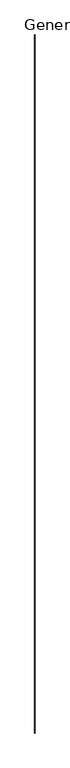
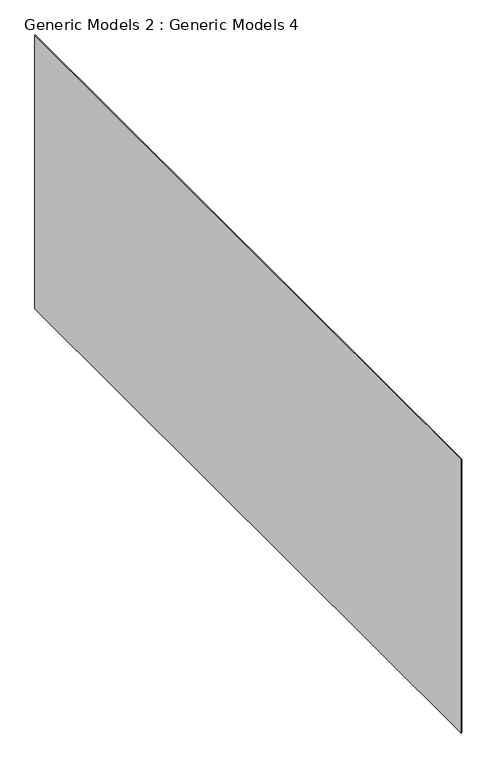
"""IFC4 building model written with IfcOpenShell, lengths in millimetres: proxy geometry, Generic Models 2 : Generic Models 4."""

from ifc_helpers import new_model, si_unit, frame, origin, place, context, project, spatial, polyline, outline, extrude, source, transform, mapped, element, save


def generic_models_2_generic_models_4_d4be96ae(model_context):
    return source(origin(), model_context, "Body", "SweptSolid", [
        extrude(outline(polyline([(593591.3576893, -527524.3545647), (593591.3576893, -584979.050959), (593565.9576893, -584979.050959), (593565.9576893, -527524.3545647), (593591.3576893, -527524.3545647)])), frame((0.0, 0.0, -2503.337634), z_axis=(0.0, 0.0, 1.0), x_axis=(1.0, 0.0, 0.0)), (0.0, 0.0, 1.0), 22488.6259865),
    ])


if __name__ == "__main__":
    model = new_model("IFC4")
    model_context = context("Model", 3, world=origin())
    ifc_project = project(units=[si_unit("LENGTHUNIT", "METRE", prefix="MILLI")], contexts=[model_context])
    site = spatial("IfcSite", under=ifc_project)
    building = spatial("IfcBuilding", under=site)
    placement = place(None, origin())
    generic_models_2_generic_models_4_shape = generic_models_2_generic_models_4_d4be96ae(model_context)
    element("IfcBuildingElementProxy", 1, Name="Generic Models 2 : Generic Models 4", ObjectType="Generic Models 2 : Generic Models 4", at=placement, inside=building, context=model_context, shape_type="MappedRepresentation", body=[
        mapped(generic_models_2_generic_models_4_shape, transform((0.0, 0.0, 0.0), x_axis=(1.0, 0.0, 0.0), y_axis=(0.0, 1.0, 0.0), z_axis=(0.0, 0.0, 1.0))),
    ])
    save(model, "model.ifc")

# Revit data of these elements
# Element 1 (IfcBuildingElementProxy, "Generic Models 2 : Generic Models 4")
#   Materials on its faces: "Air"
# Materials
#   "Air": class "Gas", colour RGB 255 255 255, transparency 1, Description = "Air", Cost = 0
